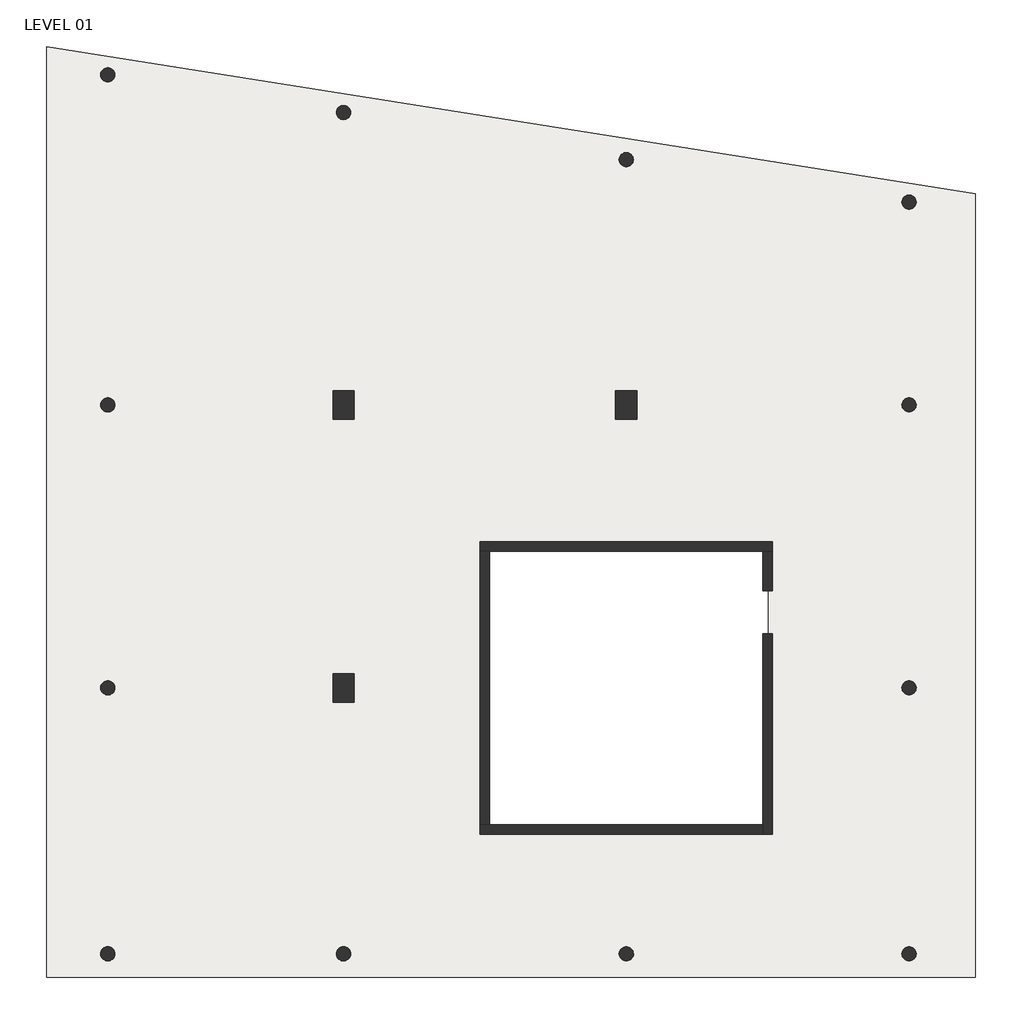
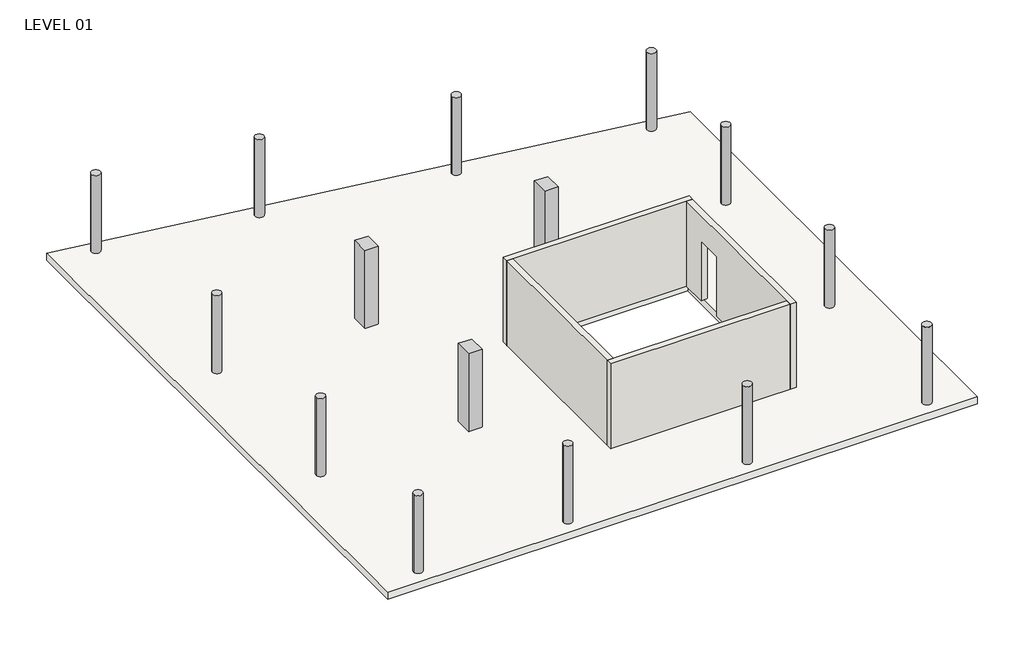
# One storey: 15 columns, 4 beams, 4 walls, 1 slab.
"""IFC4 building model written with IfcOpenShell, lengths in millimetres."""

from ifc_helpers import new_model, si_unit, point, frame, frame_2d, origin, place, context, project, spatial, polyline, circle_curve, trimmed, segment, composite_curve, outline, extrude, faceted_brep, element, save
from ifc_brep_helpers import plane_surface, revolved_surface, advanced_brep

model = new_model("IFC4")

# Units and contexts
model_context = context("Model", 3, world=origin())
ifc_project = project(units=[si_unit("LENGTHUNIT", "METRE", prefix="MILLI")], contexts=[model_context])

# Site, building, storey
site = spatial("IfcSite", under=ifc_project)
building = spatial("IfcBuilding", under=site)
storey = spatial("IfcBuildingStorey", under=building, Name="LEVEL 01", Elevation=3000.0)

# Beams
placement = place(None, origin())
element("IfcBeam", 1, ObjectType="BHm_StructuralFraming_Concrete-RectangularBeam : 300x500 DP RC BEAM", at=placement, inside=storey, context=model_context, shape_type="SweptSolid", body=[
    extrude(outline(composite_curve([segment(polyline([(-15925.1680269, 21640.7845261), (-15925.1680269, 14640.7845261)]), True, "CONTINUOUS"), segment(trimmed(circle_curve(frame_2d((-16075.1680269, 14640.7845261)), 150.0), [point((-15925.1680269, 14640.7845261))], [point((-16225.1680269, 14640.7845261))], True, "CARTESIAN"), True, "CONTINUOUS"), segment(polyline([(-16225.1680269, 14640.7845261), (-16225.1680269, 21640.7845261)]), True, "CONTINUOUS"), segment(trimmed(circle_curve(frame_2d((-16075.1680269, 21640.7845261)), 150.0), [point((-16225.1680269, 21640.7845261))], [point((-15925.1680269, 21640.7845261))], True, "CARTESIAN"), True, "CONTINUOUS")], self_intersect=False)), frame((0.0, 0.0, 2500.0), z_axis=(0.0, 0.0, 1.0), x_axis=(1.0, 0.0, 0.0)), (0.0, 0.0, 1.0), 250.0),
])
element("IfcBeam", 2, ObjectType="BHm_StructuralFraming_Concrete-RectangularBeam : 300x500 DP RC BEAM", at=placement, inside=storey, context=model_context, shape_type="AdvancedBrep", body=[
    advanced_brep(
    [(-10925.1680269, 14940.7845261, 2500.0), (-10925.1680269, 20840.7845261, 2500.0), (-10925.1680269, 20840.7845261, 2750.0), (-10925.1680269, 14940.7845261, 2750.0), (-11225.1680269, 14940.7845261, 2500.0), (-11225.1680269, 20840.7845261, 2500.0), (-11225.1680269, 14940.7845261, 2750.0), (-11225.1680269, 20840.7845261, 2750.0)],
    [
        (0, 1),
        (1, 2),
        (2, 3),
        (3, 0),
        (0, 4),
        (4, 5),
        (5, 1, circle_curve(frame((-11075.1680269, 20840.7845261, 2500.0), z_axis=(0.0, 0.0, 1.0), x_axis=(1.0, 0.0, 0.0)), 150.0)),
        (4, 6),
        (6, 7),
        (7, 5),
        (3, 6),
        (7, 2, circle_curve(frame((-11075.1680269, 20840.7845261, 2750.0), z_axis=(0.0, 0.0, 1.0), x_axis=(1.0, 0.0, 0.0)), 150.0)),
    ],
    [
        plane_surface(frame((-10925.1680269, 20691.7845261, 3000.0), z_axis=(1.0, 0.0, 0.0), x_axis=(0.0, -1.0, 0.0))),
        plane_surface(frame((-10925.1680269, 20691.7845261, 2500.0), z_axis=(0.0, 0.0, -1.0), x_axis=(0.0, -1.0, 0.0))),
        plane_surface(frame((-11225.1680269, 20691.7845261, 2500.0), z_axis=(-1.0, 0.0, 0.0), x_axis=(0.0, -1.0, 0.0))),
        plane_surface(frame((-10850.1680269, 14940.7845261, 3000.0), z_axis=(0.0, -1.0, 0.0), x_axis=(0.0, 0.0, -1.0))),
        revolved_surface(polyline([(-10925.1680269, 20840.7845261, 2750.0), (-10925.1680269, 20840.7845261, 2500.0)]), (-11075.1680269, 20840.7845261, 0.0), (0.0, 0.0, 1.0)),
        plane_surface(frame((2324.8319731, 15140.7845261, 2750.0), z_axis=(0.0, 0.0, 1.0), x_axis=(0.0, -1.0, 0.0))),
    ],
    [
        (0, [[1, 2, 3, 4]]),
        (1, [[-1, 5, 6, 7]]),
        (2, [[-6, 8, 9, 10]]),
        (3, [[-5, -4, 11, -8]]),
        (4, [[-7, -10, 12, -2]]),
        (5, [[-3, -12, -9, -11]]),
    ],
),
])
element("IfcBeam", 3, ObjectType="BHm_StructuralFraming_Concrete-RectangularBeam : 300x500 DP RC BEAM", at=placement, inside=storey, context=model_context, shape_type="SweptSolid", body=[
    extrude(outline(composite_curve([segment(polyline([(-4925.1680269, 19840.7845261), (-4925.1680269, 14940.7845261), (-5225.1680269, 14940.7845261), (-5225.1680269, 19840.7845261)]), True, "CONTINUOUS"), segment(trimmed(circle_curve(frame_2d((-5075.1680269, 19840.7845261)), 150.0), [point((-5225.1680269, 19840.7845261))], [point((-4925.1680269, 19840.7845261))], True, "CARTESIAN"), True, "CONTINUOUS")], self_intersect=False)), frame((0.0, 0.0, 2500.0), z_axis=(0.0, 0.0, 1.0), x_axis=(1.0, 0.0, 0.0)), (0.0, 0.0, 1.0), 250.0),
])
element("IfcBeam", 4, ObjectType="BHm_StructuralFraming_Concrete-RectangularBeam : 300x500 DP RC BEAM", at=placement, inside=storey, context=model_context, shape_type="SweptSolid", body=[
    extrude(outline(composite_curve([segment(polyline([(1074.8319731, 18940.7845261), (1074.8319731, 14640.7845261)]), True, "CONTINUOUS"), segment(trimmed(circle_curve(frame_2d((924.8319731, 14640.7845261)), 150.0), [point((1074.8319731, 14640.7845261))], [point((774.8319731, 14640.7845261))], True, "CARTESIAN"), True, "CONTINUOUS"), segment(polyline([(774.8319731, 14640.7845261), (774.8319731, 18940.7845261)]), True, "CONTINUOUS"), segment(trimmed(circle_curve(frame_2d((924.8319731, 18940.7845261)), 150.0), [point((774.8319731, 18940.7845261))], [point((1074.8319731, 18940.7845261))], True, "CARTESIAN"), True, "CONTINUOUS")], self_intersect=False)), frame((0.0, 0.0, 2500.0), z_axis=(0.0, 0.0, 1.0), x_axis=(1.0, 0.0, 0.0)), (0.0, 0.0, 1.0), 250.0),
])

# Columns
element("IfcColumn", 5, ObjectType="BHm_StructuralColumns_ConcreteRound : 300 Ø RC COL", at=placement, inside=storey, context=model_context, shape_type="SweptSolid", body=[
    extrude(outline(composite_curve([segment(trimmed(circle_curve(frame_2d((-11075.1680269, 3000.0)), 150.0), [point((-11225.1680269, 3000.0))], [point((-10925.1680269, 3000.0))], False, "CARTESIAN"), True, "CONTINUOUS"), segment(trimmed(circle_curve(frame_2d((-11075.1680269, 3000.0)), 150.0), [point((-10925.1680269, 3000.0))], [point((-11225.1680269, 3000.0))], False, "CARTESIAN"), True, "CONTINUOUS")], self_intersect=False)), frame((0.0, 0.0, 3000.0), z_axis=(0.0, 0.0, 1.0), x_axis=(1.0, 0.0, 0.0)), (0.0, 0.0, 1.0), 2750.0),
])
element("IfcColumn", 6, ObjectType="BHm_StructuralColumns_ConcreteRound : 300 Ø RC COL", at=placement, inside=storey, context=model_context, shape_type="SweptSolid", body=[
    extrude(outline(composite_curve([segment(trimmed(circle_curve(frame_2d((-5075.1680269, 3000.0)), 150.0), [point((-5225.1680269, 3000.0))], [point((-4925.1680269, 3000.0))], False, "CARTESIAN"), True, "CONTINUOUS"), segment(trimmed(circle_curve(frame_2d((-5075.1680269, 3000.0)), 150.0), [point((-4925.1680269, 3000.0))], [point((-5225.1680269, 3000.0))], False, "CARTESIAN"), True, "CONTINUOUS")], self_intersect=False)), frame((0.0, 0.0, 3000.0), z_axis=(0.0, 0.0, 1.0), x_axis=(1.0, 0.0, 0.0)), (0.0, 0.0, 1.0), 2750.0),
])
element("IfcColumn", 7, ObjectType="BHm_StructuralColumns_ConcreteRound : 300 Ø RC COL", at=placement, inside=storey, context=model_context, shape_type="SweptSolid", body=[
    extrude(outline(composite_curve([segment(trimmed(circle_curve(frame_2d((924.8319731, 14640.7845261)), 150.0), [point((774.8319731, 14640.7845261))], [point((1074.8319731, 14640.7845261))], False, "CARTESIAN"), True, "CONTINUOUS"), segment(trimmed(circle_curve(frame_2d((924.8319731, 14640.7845261)), 150.0), [point((1074.8319731, 14640.7845261))], [point((774.8319731, 14640.7845261))], False, "CARTESIAN"), True, "CONTINUOUS")], self_intersect=False)), frame((0.0, 0.0, 3000.0), z_axis=(0.0, 0.0, 1.0), x_axis=(1.0, 0.0, 0.0)), (0.0, 0.0, 1.0), 2750.0),
])
element("IfcColumn", 8, ObjectType="BHm_StructuralColumns_ConcreteRound : 300 Ø RC COL", at=placement, inside=storey, context=model_context, shape_type="SweptSolid", body=[
    extrude(outline(composite_curve([segment(trimmed(circle_curve(frame_2d((924.8319731, 8640.7845261)), 150.0), [point((774.8319731, 8640.7845261))], [point((1074.8319731, 8640.7845261))], False, "CARTESIAN"), True, "CONTINUOUS"), segment(trimmed(circle_curve(frame_2d((924.8319731, 8640.7845261)), 150.0), [point((1074.8319731, 8640.7845261))], [point((774.8319731, 8640.7845261))], False, "CARTESIAN"), True, "CONTINUOUS")], self_intersect=False)), frame((0.0, 0.0, 3000.0), z_axis=(0.0, 0.0, 1.0), x_axis=(1.0, 0.0, 0.0)), (0.0, 0.0, 1.0), 2750.0),
])
element("IfcColumn", 9, ObjectType="BHm_StructuralColumns_ConcreteRound : 300 Ø RC COL", at=placement, inside=storey, context=model_context, shape_type="SweptSolid", body=[
    extrude(outline(composite_curve([segment(trimmed(circle_curve(frame_2d((924.8319731, 3000.0)), 150.0), [point((774.8319731, 3000.0))], [point((1074.8319731, 3000.0))], False, "CARTESIAN"), True, "CONTINUOUS"), segment(trimmed(circle_curve(frame_2d((924.8319731, 3000.0)), 150.0), [point((1074.8319731, 3000.0))], [point((774.8319731, 3000.0))], False, "CARTESIAN"), True, "CONTINUOUS")], self_intersect=False)), frame((0.0, 0.0, 3000.0), z_axis=(0.0, 0.0, 1.0), x_axis=(1.0, 0.0, 0.0)), (0.0, 0.0, 1.0), 2750.0),
])
element("IfcColumn", 10, ObjectType="BHm_StructuralColumns_ConcreteRound : 300 Ø RC COL", at=placement, inside=storey, context=model_context, shape_type="SweptSolid", body=[
    extrude(outline(composite_curve([segment(trimmed(circle_curve(frame_2d((-16075.1680269, 14640.7845261)), 150.0), [point((-16225.1680269, 14640.7845261))], [point((-15925.1680269, 14640.7845261))], False, "CARTESIAN"), True, "CONTINUOUS"), segment(trimmed(circle_curve(frame_2d((-16075.1680269, 14640.7845261)), 150.0), [point((-15925.1680269, 14640.7845261))], [point((-16225.1680269, 14640.7845261))], False, "CARTESIAN"), True, "CONTINUOUS")], self_intersect=False)), frame((0.0, 0.0, 3000.0), z_axis=(0.0, 0.0, 1.0), x_axis=(1.0, 0.0, 0.0)), (0.0, 0.0, 1.0), 2750.0),
])
element("IfcColumn", 11, ObjectType="BHm_StructuralColumns_ConcreteRound : 300 Ø RC COL", at=placement, inside=storey, context=model_context, shape_type="SweptSolid", body=[
    extrude(outline(composite_curve([segment(trimmed(circle_curve(frame_2d((-16075.1680269, 8640.7845261)), 150.0), [point((-16225.1680269, 8640.7845261))], [point((-15925.1680269, 8640.7845261))], False, "CARTESIAN"), True, "CONTINUOUS"), segment(trimmed(circle_curve(frame_2d((-16075.1680269, 8640.7845261)), 150.0), [point((-15925.1680269, 8640.7845261))], [point((-16225.1680269, 8640.7845261))], False, "CARTESIAN"), True, "CONTINUOUS")], self_intersect=False)), frame((0.0, 0.0, 3000.0), z_axis=(0.0, 0.0, 1.0), x_axis=(1.0, 0.0, 0.0)), (0.0, 0.0, 1.0), 2750.0),
])
element("IfcColumn", 12, ObjectType="BHm_StructuralColumns_ConcreteRound : 300 Ø RC COL", at=placement, inside=storey, context=model_context, shape_type="SweptSolid", body=[
    extrude(outline(composite_curve([segment(trimmed(circle_curve(frame_2d((-16075.1680269, 3000.0)), 150.0), [point((-16225.1680269, 3000.0))], [point((-15925.1680269, 3000.0))], False, "CARTESIAN"), True, "CONTINUOUS"), segment(trimmed(circle_curve(frame_2d((-16075.1680269, 3000.0)), 150.0), [point((-15925.1680269, 3000.0))], [point((-16225.1680269, 3000.0))], False, "CARTESIAN"), True, "CONTINUOUS")], self_intersect=False)), frame((0.0, 0.0, 3000.0), z_axis=(0.0, 0.0, 1.0), x_axis=(1.0, 0.0, 0.0)), (0.0, 0.0, 1.0), 2750.0),
])
element("IfcColumn", 13, ObjectType="BHm_StructuralColumns_ConcreteRound : 300 Ø RC COL", at=placement, inside=storey, context=model_context, shape_type="SweptSolid", body=[
    extrude(outline(composite_curve([segment(trimmed(circle_curve(frame_2d((-11075.1680269, 20840.7845261)), 150.0), [point((-11225.1680269, 20840.7845261))], [point((-10925.1680269, 20840.7845261))], False, "CARTESIAN"), True, "CONTINUOUS"), segment(trimmed(circle_curve(frame_2d((-11075.1680269, 20840.7845261)), 150.0), [point((-10925.1680269, 20840.7845261))], [point((-11225.1680269, 20840.7845261))], False, "CARTESIAN"), True, "CONTINUOUS")], self_intersect=False)), frame((0.0, 0.0, 3000.0), z_axis=(0.0, 0.0, 1.0), x_axis=(1.0, 0.0, 0.0)), (0.0, 0.0, 1.0), 2750.0),
])
element("IfcColumn", 14, ObjectType="BHm_StructuralColumns_ConcreteRound : 300 Ø RC COL", at=placement, inside=storey, context=model_context, shape_type="SweptSolid", body=[
    extrude(outline(composite_curve([segment(trimmed(circle_curve(frame_2d((-5075.1680269, 19840.7845261)), 150.0), [point((-5225.1680269, 19840.7845261))], [point((-4925.1680269, 19840.7845261))], False, "CARTESIAN"), True, "CONTINUOUS"), segment(trimmed(circle_curve(frame_2d((-5075.1680269, 19840.7845261)), 150.0), [point((-4925.1680269, 19840.7845261))], [point((-5225.1680269, 19840.7845261))], False, "CARTESIAN"), True, "CONTINUOUS")], self_intersect=False)), frame((0.0, 0.0, 3000.0), z_axis=(0.0, 0.0, 1.0), x_axis=(1.0, 0.0, 0.0)), (0.0, 0.0, 1.0), 2750.0),
])
element("IfcColumn", 15, ObjectType="BHm_StructuralColumns_ConcreteRound : 300 Ø RC COL", at=placement, inside=storey, context=model_context, shape_type="SweptSolid", body=[
    extrude(outline(composite_curve([segment(trimmed(circle_curve(frame_2d((924.8319731, 18940.7845261)), 150.0), [point((774.8319731, 18940.7845261))], [point((1074.8319731, 18940.7845261))], False, "CARTESIAN"), True, "CONTINUOUS"), segment(trimmed(circle_curve(frame_2d((924.8319731, 18940.7845261)), 150.0), [point((1074.8319731, 18940.7845261))], [point((774.8319731, 18940.7845261))], False, "CARTESIAN"), True, "CONTINUOUS")], self_intersect=False)), frame((0.0, 0.0, 3000.0), z_axis=(0.0, 0.0, 1.0), x_axis=(1.0, 0.0, 0.0)), (0.0, 0.0, 1.0), 2750.0),
])
element("IfcColumn", 16, ObjectType="BHm_StructuralColumns_ConcreteRound : 300 Ø RC COL", at=placement, inside=storey, context=model_context, shape_type="SweptSolid", body=[
    extrude(outline(composite_curve([segment(trimmed(circle_curve(frame_2d((-16075.1680269, 21640.7845261)), 150.0), [point((-16225.1680269, 21640.7845261))], [point((-15925.1680269, 21640.7845261))], False, "CARTESIAN"), True, "CONTINUOUS"), segment(trimmed(circle_curve(frame_2d((-16075.1680269, 21640.7845261)), 150.0), [point((-15925.1680269, 21640.7845261))], [point((-16225.1680269, 21640.7845261))], False, "CARTESIAN"), True, "CONTINUOUS")], self_intersect=False)), frame((0.0, 0.0, 3000.0), z_axis=(0.0, 0.0, 1.0), x_axis=(1.0, 0.0, 0.0)), (0.0, 0.0, 1.0), 2750.0),
])
element("IfcColumn", 17, ObjectType="BHm_StructuralColumns_ConcreteRectangular : 450x600 RC COL", at=placement, inside=storey, context=model_context, shape_type="SweptSolid", body=[
    extrude(outline(polyline([(-10850.1680269, 14940.7845261), (-10850.1680269, 14340.7845261), (-11300.1680269, 14340.7845261), (-11300.1680269, 14940.7845261), (-10850.1680269, 14940.7845261)])), frame((0.0, 0.0, 3000.0), z_axis=(0.0, 0.0, 1.0), x_axis=(1.0, 0.0, 0.0)), (0.0, 0.0, 1.0), 2750.0),
])
element("IfcColumn", 18, ObjectType="BHm_StructuralColumns_ConcreteRectangular : 450x600 RC COL", at=placement, inside=storey, context=model_context, shape_type="SweptSolid", body=[
    extrude(outline(polyline([(-10850.1680269, 8940.7845261), (-10850.1680269, 8340.7845261), (-11300.1680269, 8340.7845261), (-11300.1680269, 8940.7845261), (-10850.1680269, 8940.7845261)])), frame((0.0, 0.0, 3000.0), z_axis=(0.0, 0.0, 1.0), x_axis=(1.0, 0.0, 0.0)), (0.0, 0.0, 1.0), 2750.0),
])
element("IfcColumn", 19, ObjectType="BHm_StructuralColumns_ConcreteRectangular : 450x600 RC COL", at=placement, inside=storey, context=model_context, shape_type="SweptSolid", body=[
    extrude(outline(polyline([(-4850.1680269, 14940.7845261), (-4850.1680269, 14340.7845261), (-5300.1680269, 14340.7845261), (-5300.1680269, 14940.7845261), (-4850.1680269, 14940.7845261)])), frame((0.0, 0.0, 3000.0), z_axis=(0.0, 0.0, 1.0), x_axis=(1.0, 0.0, 0.0)), (0.0, 0.0, 1.0), 2750.0),
])

# Slab
element("IfcSlab", 20, ObjectType="250 THK RC SLAB", at=placement, inside=storey, context=model_context, shape_type="SweptSolid", body=[
    extrude(outline(polyline([(2324.8319731, 19120.6110517), (2324.8319731, 2500.0), (-17375.1680269, 2500.0), (-17375.1680269, 22240.7845261), (2324.8319731, 19120.6110517)]), holes=[polyline([(-2075.1680269, 11640.7845261), (-8075.1680269, 11640.7845261), (-8075.1680269, 5640.7845261), (-2075.1680269, 5640.7845261), (-2075.1680269, 11640.7845261)])]), frame((0.0, 0.0, 2750.0), z_axis=(0.0, 0.0, 1.0), x_axis=(1.0, 0.0, 0.0)), (0.0, 0.0, 1.0), 250.0),
])

# Walls
element("IfcWall", 21, ObjectType="200 THK R.C. WALL", at=placement, inside=storey, context=model_context, shape_type="Brep", body=[
    faceted_brep([(-8175.1680269, 11540.7845261, 3000.0), (-7975.1680269, 11540.7845261, 3000.0), (-2175.1680269, 11540.7845261, 3000.0), (-1975.1680269, 11540.7845261, 3000.0), (-1975.1680269, 11540.7845261, 6000.0), (-2175.1680269, 11540.7845261, 6000.0), (-7975.1680269, 11540.7845261, 6000.0), (-8175.1680269, 11540.7845261, 6000.0), (-8175.1680269, 11740.7845261, 3000.0), (-8175.1680269, 11740.7845261, 6000.0), (-1975.1680269, 11740.7845261, 6000.0), (-1975.1680269, 11740.7845261, 3000.0)], [[[0, 1, 2, 3, 4, 5, 6, 7]], [[8, 9, 10, 11]], [[3, 2, 1, 0, 8, 11]], [[7, 6, 5, 4, 10, 9]], [[4, 3, 11, 10]], [[0, 7, 9, 8]]]),
])
element("IfcWall", 22, ObjectType="200 THK R.C. WALL", at=placement, inside=storey, context=model_context, shape_type="Brep", body=[
    faceted_brep([(-2175.1680269, 11540.7845261, 3000.0), (-2175.1680269, 10698.2845261, 3000.0), (-2175.1680269, 10698.2845261, 5100.0), (-2175.1680269, 9783.2845261, 5100.0), (-2175.1680269, 9783.2845261, 3000.0), (-2175.1680269, 5740.7845261, 3000.0), (-2175.1680269, 5540.7845261, 3000.0), (-2175.1680269, 5540.7845261, 6000.0), (-2175.1680269, 5740.7845261, 6000.0), (-2175.1680269, 11540.7845261, 6000.0), (-1975.1680269, 10698.2845261, 5100.0), (-1975.1680269, 10698.2845261, 3000.0), (-1975.1680269, 11540.7845261, 3000.0), (-1975.1680269, 11540.7845261, 6000.0), (-1975.1680269, 5540.7845261, 6000.0), (-1975.1680269, 5540.7845261, 3000.0), (-1975.1680269, 9783.2845261, 3000.0), (-1975.1680269, 9783.2845261, 5100.0)], [[[0, 1, 2, 3, 4, 5, 6, 7, 8, 9]], [[10, 11, 12, 13, 14, 15, 16, 17]], [[16, 15, 6, 5, 4]], [[12, 11, 1, 0]], [[9, 8, 7, 14, 13]], [[0, 9, 13, 12]], [[7, 6, 15, 14]], [[4, 3, 17, 16]], [[2, 1, 11, 10]], [[3, 2, 10, 17]]]),
])
element("IfcWall", 23, ObjectType="200 THK R.C. WALL", at=placement, inside=storey, context=model_context, shape_type="Brep", body=[
    faceted_brep([(-2175.1680269, 5740.7845261, 3000.0), (-7975.1680269, 5740.7845261, 3000.0), (-8175.1680269, 5740.7845261, 3000.0), (-8175.1680269, 5740.7845261, 6000.0), (-7975.1680269, 5740.7845261, 6000.0), (-2175.1680269, 5740.7845261, 6000.0), (-2175.1680269, 5540.7845261, 3000.0), (-2175.1680269, 5540.7845261, 6000.0), (-8175.1680269, 5540.7845261, 6000.0), (-8175.1680269, 5540.7845261, 3000.0)], [[[0, 1, 2, 3, 4, 5]], [[6, 7, 8, 9]], [[2, 1, 0, 6, 9]], [[5, 4, 3, 8, 7]], [[0, 5, 7, 6]], [[3, 2, 9, 8]]]),
])
element("IfcWall", 24, ObjectType="200 THK R.C. WALL", at=placement, inside=storey, context=model_context, shape_type="SweptSolid", body=[
    extrude(outline(polyline([(-7975.1680269, 11540.7845261), (-7975.1680269, 5740.7845261), (-8175.1680269, 5740.7845261), (-8175.1680269, 11540.7845261), (-7975.1680269, 11540.7845261)])), frame((0.0, 0.0, 3000.0), z_axis=(0.0, 0.0, 1.0), x_axis=(1.0, 0.0, 0.0)), (0.0, 0.0, 1.0), 3000.0),
])

save(model, "model.ifc")

# Revit data of these elements
# Type "BHm_StructuralFraming_Concrete-RectangularBeam : 300x500 DP RC BEAM"
#   Keynote = "E"
#   BHE_Width = 300.000 mm
#   BHE_Length [instance default] = 1524.000 mm
#   BHE_Height = 500.000 mm
#   Length [instance default] = 1524.000 mm
#   b = 300.000 mm
#   h = 500.000 mm
#   Structural Material [instance default] = none
#   Assembly Code = ""
# Type "BHm_StructuralColumns_ConcreteRound : 300 Ø RC COL"
#   Keynote = "E"
#   b = 300.000 mm
#   BHE_Length [instance default] = 2500.000 mm
#   BHE_Diameter = 300.000 mm
#   Structural Material [instance default] = none
# Type "BHm_StructuralColumns_ConcreteRectangular : 450x600 RC COL"
#   Keynote = "E"
#   b = 450.000 mm
#   h = 600.000 mm
#   BHE_Width = 450.000 mm
#   BHE_Length [instance default] = 2500.000 mm
#   BHE_Height = 600.000 mm
#   Structural Material [instance default] = none
# Type "250 THK RC SLAB"
#   Function = 0
#   Layers, outside or top first: 250.000 mm "BHE_Concrete - Cast In-Place" (function 1)
# Type "200 THK R.C. WALL"
#   Layers, outside or top first: 200.000 mm "BHE_Concrete - Cast In-Place" (function 1)
# Element 1 (IfcBeam, "BHm_StructuralFraming_Concrete-RectangularBeam : 300x500 DP RC BEAM")
#   Comments = ""
#   BHE_Length = 7000.000 mm
#   Structural Material = none
#   Phase Created = New Construction
#   Materials on its faces: "BHE_Concrete - Cast In-Place"
# Element 2 (IfcBeam, "BHm_StructuralFraming_Concrete-RectangularBeam : 300x500 DP RC BEAM")
#   Comments = ""
#   BHE_Length = 6200.000 mm
#   Structural Material = none
#   Phase Created = New Construction
#   Materials on its faces: "BHE_Concrete - Cast In-Place"
# Element 3 (IfcBeam, "BHm_StructuralFraming_Concrete-RectangularBeam : 300x500 DP RC BEAM")
#   Comments = ""
#   BHE_Length = 5200.000 mm
#   Structural Material = none
#   Phase Created = New Construction
#   Materials on its faces: "BHE_Concrete - Cast In-Place"
# Element 4 (IfcBeam, "BHm_StructuralFraming_Concrete-RectangularBeam : 300x500 DP RC BEAM")
#   Comments = ""
#   BHE_Length = 4300.000 mm
#   Structural Material = none
#   Phase Created = New Construction
#   Materials on its faces: "BHE_Concrete - Cast In-Place"
# Elements 5, 6, 7, 8, 9, 10, 11, 12, 13, 14, 15, 16 (IfcColumn, "BHm_StructuralColumns_ConcreteRound : 300 Ø RC COL")
#   Comments = ""
#   Structural Material = none
#   Phase Created = New Construction
#   Materials on its faces: "BHE_Concrete - Cast In-Place"
# Elements 17, 18, 19 (IfcColumn, "BHm_StructuralColumns_ConcreteRectangular : 450x600 RC COL")
#   Comments = ""
#   Structural Material = none
#   Phase Created = New Construction
#   Materials on its faces: "BHE_Concrete - Cast In-Place"
# Element 20 (IfcSlab, "250 THK RC SLAB")
#   Comments = ""
#   built-in parameter 1001955 = -0.15708 (stored number, unit not read)
#   Height Offset From Level = 0.000 mm
#   built-in parameter 1001954 = 1
#   Phase Created = New Construction
#   Materials on its faces: "BHE_Concrete - Cast In-Place"
# Elements 21, 22, 23, 24 (IfcWall, "200 THK R.C. WALL")
#   Comments = ""
#   Top Offset = 0.000 mm
#   Base Offset = 0.000 mm
#   wall height = 3000.000 mm
#   Phase Created = New Construction
#   Base Constraint = LEVEL 01
#   Top Constraint = LEVEL 02
#   Materials on its faces: "BHE_Concrete - Cast In-Place"
# Materials
#   "BHE_Concrete - Cast In-Place": class "Concrete", colour RGB 192 192 192, transparency 0, Cost = 0
